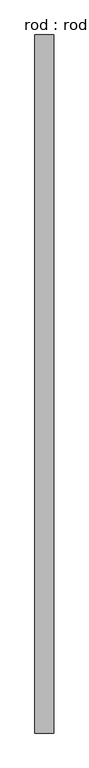
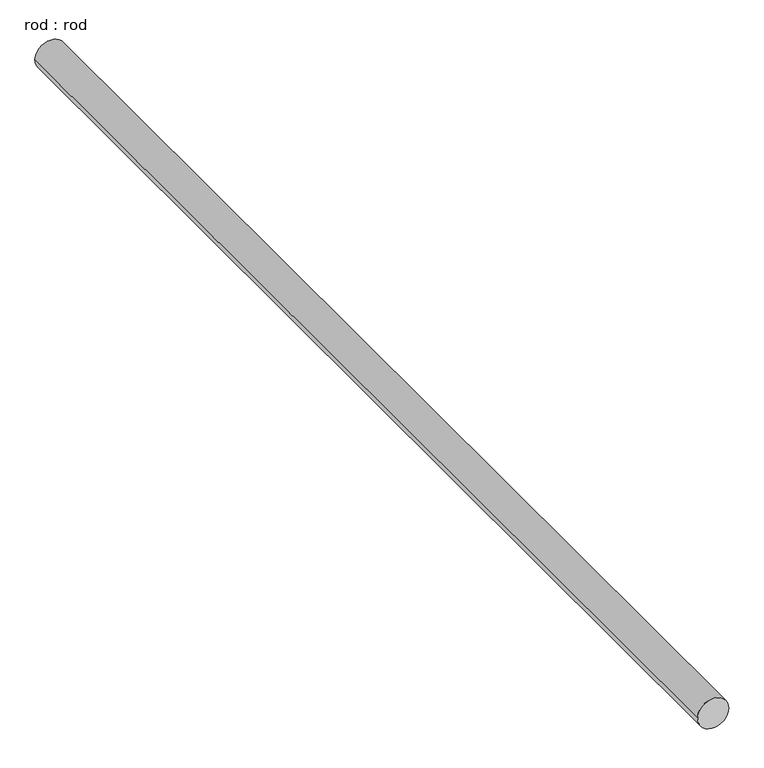
"""IFC4 building model written with IfcOpenShell, lengths in millimetres: proxy geometry, rod : rod."""

from ifc_helpers import new_model, si_unit, point, frame, frame_2d, origin, place, context, project, spatial, circle_curve, trimmed, segment, composite_curve, outline, extrude, source, transform, mapped, element, save


def rod_rod_ec035f66(model_context):
    return source(origin(), model_context, "Body", "SweptSolid", [
        extrude(outline(composite_curve([segment(trimmed(circle_curve(frame_2d((0.0108462, 0.0)), 200.0), [point((0.0108462, 200.0))], [point((0.0108462, -200.0))], False, "CARTESIAN"), True, "CONTINUOUS"), segment(trimmed(circle_curve(frame_2d((0.0108462, 0.0)), 200.0), [point((0.0108462, -200.0))], [point((0.0108462, 200.0))], False, "CARTESIAN"), True, "CONTINUOUS")], self_intersect=False)), frame((0.0, -3264.4142418, 0.0), z_axis=(0.0, 1.0, 0.0), x_axis=(0.0, 0.0, 1.0)), (0.0, 0.0, 1.0), 14714.2857143),
    ])


if __name__ == "__main__":
    model = new_model("IFC4")
    model_context = context("Model", 3, world=origin())
    ifc_project = project(units=[si_unit("LENGTHUNIT", "METRE", prefix="MILLI")], contexts=[model_context])
    site = spatial("IfcSite", under=ifc_project)
    building = spatial("IfcBuilding", under=site)
    placement = place(None, origin())
    rod_rod_shape = rod_rod_ec035f66(model_context)
    element("IfcBuildingElementProxy", 1, Name="rod : rod", ObjectType="rod : rod", at=placement, inside=building, context=model_context, shape_type="MappedRepresentation", body=[
        mapped(rod_rod_shape, transform((0.0, 0.0, 0.0), x_axis=(1.0, 0.0, 0.0), y_axis=(0.0, 1.0, 0.0), z_axis=(0.0, 0.0, 1.0))),
    ])
    save(model, "model.ifc")

# Revit data of these elements
# Type "rod : rod"
#   Default Elevation = 0
